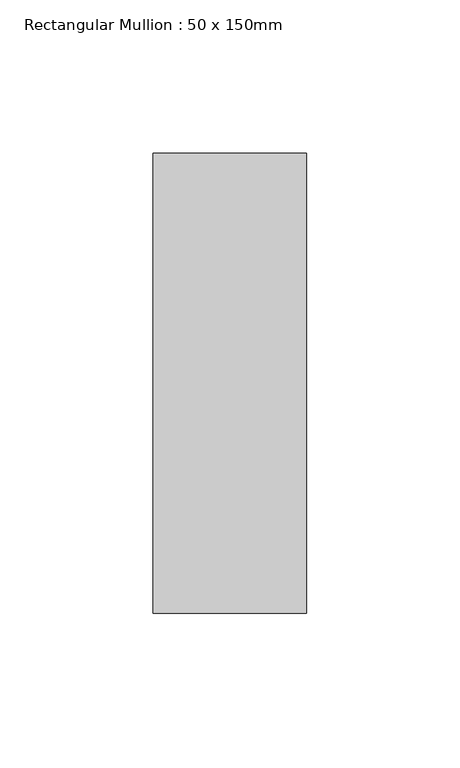
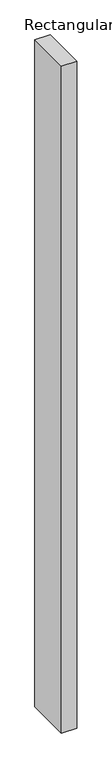
"""IFC4 building model written with IfcOpenShell, lengths in millimetres: member geometry, Rectangular Mullion : 50 x 150mm."""

import ifcopenshell
import ifcopenshell.guid

model = None  # the IFC model being written
_history = None  # IfcOwnerHistory: only IFC2X3 demands one
_inside = {}  # id of a spatial element -> (the spatial element, [elements in it])
_under = {}  # id of a project, library or spatial element -> (it, [spatial elements below it])
_declared = {}  # id of a project -> (the project, [libraries it declares])
_typed = {}  # id of a type object -> (the type object, [elements of that type])
_made_of = {}  # id of a material, layer set ... -> (it, [elements and type objects made of it])


def new_model(schema):
    """Start an empty IFC model of exactly this schema.

    Asked for "IFC4X3", IfcOpenShell would pick the latest addendum, in which some entities
    have other attributes; the version numbers below select the first issue.
    IFC2X3 requires an IfcOwnerHistory on every rooted entity: one is made here for all.
    """
    global model, _history
    if schema == "IFC4X3":
        model = ifcopenshell.file(schema_version=(4, 3, 0, 0))
    else:
        model = ifcopenshell.file(schema=schema)
    _inside.clear()
    _under.clear()
    _declared.clear()
    _typed.clear()
    _made_of.clear()
    _history = None
    if model.schema == "IFC2X3":
        org = make("IfcOrganization", Name="unknown")
        user = make(
            "IfcPersonAndOrganization",
            ThePerson=make("IfcPerson", FamilyName="unknown"),
            TheOrganization=org,
        )
        app = make(
            "IfcApplication",
            ApplicationDeveloper=org,
            Version="unknown",
            ApplicationFullName="unknown",
            ApplicationIdentifier="unknown",
        )
        _history = make(
            "IfcOwnerHistory",
            OwningUser=user,
            OwningApplication=app,
            ChangeAction="ADDED",
            CreationDate=0,
        )
    return model


def make(cls, **values):
    """One entity of the class cls with the attributes given. An attribute that is None is left unset."""
    return model.create_entity(
        cls, **{name: value for name, value in values.items() if value is not None}
    )


def rooted(cls, **values):
    """An entity with a GlobalId (a new one), such as an element, a storey or a relation."""
    return make(cls, GlobalId=ifcopenshell.guid.new(), OwnerHistory=_history, **values)


def si_unit(unit_type, name, prefix=None):
    """IfcSIUnit, for example si_unit("LENGTHUNIT", "METRE", prefix="MILLI")."""
    return make("IfcSIUnit", UnitType=unit_type, Prefix=prefix, Name=name)


def assignment(units):
    """IfcUnitAssignment: the units of a project."""
    return None if units is None else make("IfcUnitAssignment", Units=units)


def point(xyz):
    """IfcCartesianPoint."""
    return None if xyz is None else make("IfcCartesianPoint", Coordinates=xyz)


def direction(xyz):
    """IfcDirection."""
    return None if xyz is None else make("IfcDirection", DirectionRatios=xyz)


def frame(location, z_axis=None, x_axis=None):
    """IfcAxis2Placement3D, a coordinate frame: its origin and axes. An axis left out is left unset."""
    return make(
        "IfcAxis2Placement3D",
        Location=point(location),
        Axis=direction(z_axis),
        RefDirection=direction(x_axis),
    )


def origin():
    """The frame at (0, 0, 0) with its axes left unset."""
    return frame((0.0, 0.0, 0.0))


def place(relative_to, where):
    """IfcLocalPlacement: puts the frame where relative to a parent placement (None: the world)."""
    return make(
        "IfcLocalPlacement", PlacementRelTo=relative_to, RelativePlacement=where
    )


def context(
    kind, dimensions, precision=None, world=None, true_north=None, identifier=None
):
    """IfcGeometricRepresentationContext, for example the 3D "Model" context."""
    return make(
        "IfcGeometricRepresentationContext",
        ContextIdentifier=identifier,
        ContextType=kind,
        CoordinateSpaceDimension=dimensions,
        Precision=precision,
        WorldCoordinateSystem=world,
        TrueNorth=true_north,
    )


def project(units=None, contexts=None):
    """IfcProject with its units and contexts."""
    return rooted(
        "IfcProject",
        Name="project",
        RepresentationContexts=contexts,
        UnitsInContext=assignment(units),
    )


def spatial(cls, under=None, at=None, **own):
    """A site, building, storey or space (cls), placed at a placement, below another one or the project."""
    s = rooted(cls, ObjectPlacement=at, **own)
    if under is not None:
        _under.setdefault(under.id(), (under, []))[1].append(s)
    return s


def polyline(points):
    """IfcPolyline through the points."""
    return make("IfcPolyline", Points=[point(p) for p in points])


def outline(outer, holes=None, kind="AREA"):
    """IfcArbitraryClosedProfileDef: a profile drawn as a closed curve; with holes, ...WithVoids."""
    if holes is None:
        return make("IfcArbitraryClosedProfileDef", ProfileType=kind, OuterCurve=outer)
    return make(
        "IfcArbitraryProfileDefWithVoids",
        ProfileType=kind,
        OuterCurve=outer,
        InnerCurves=holes,
    )


def extrude(swept, where, along, depth):
    """IfcExtrudedAreaSolid: the profile swept, set in the frame where, extruded along a direction by depth."""
    return make(
        "IfcExtrudedAreaSolid",
        SweptArea=swept,
        Position=where,
        ExtrudedDirection=direction(along),
        Depth=depth,
    )


def shape(context_of_items, identifier, shape_type, items):
    """IfcShapeRepresentation: the items that make up one representation, for example the "Body"."""
    return make(
        "IfcShapeRepresentation",
        ContextOfItems=context_of_items,
        RepresentationIdentifier=identifier,
        RepresentationType=shape_type,
        Items=items,
    )


def source(mapping_origin, context_of_items, identifier, shape_type, items):
    """IfcRepresentationMap: a shape defined once, which mapped items show again and again."""
    return make(
        "IfcRepresentationMap",
        MappingOrigin=mapping_origin,
        MappedRepresentation=shape(context_of_items, identifier, shape_type, items),
    )


def transform(
    local_origin,
    x_axis=None,
    y_axis=None,
    z_axis=None,
    scale=None,
    scale2=None,
    scale3=None,
    uniform=True,
):
    """IfcCartesianTransformationOperator3D, or its non-uniform kind. x_axis, y_axis, z_axis: its Axis1, 2, 3."""
    if uniform:
        return make(
            "IfcCartesianTransformationOperator3D",
            Axis1=direction(x_axis),
            Axis2=direction(y_axis),
            LocalOrigin=point(local_origin),
            Scale=scale,
            Axis3=direction(z_axis),
        )
    return make(
        "IfcCartesianTransformationOperator3DnonUniform",
        Axis1=direction(x_axis),
        Axis2=direction(y_axis),
        LocalOrigin=point(local_origin),
        Scale=scale,
        Axis3=direction(z_axis),
        Scale2=scale2,
        Scale3=scale3,
    )


def mapped(mapping_source, mapping_target):
    """IfcMappedItem: shows the shape of a source again, moved by a transform."""
    return make(
        "IfcMappedItem", MappingSource=mapping_source, MappingTarget=mapping_target
    )


def made_of(thing, what):
    """Note that an element or type object is made of a material, layer set ...; save() writes the relation."""
    if what is not None:
        _made_of.setdefault(what.id(), (what, []))[1].append(thing)
    return thing


def element(
    cls,
    number,
    at=None,
    inside=None,
    cuts=None,
    type_object=None,
    material=None,
    context=None,
    identifier="Body",
    shape_type=None,
    held_by="IfcProductDefinitionShape",
    body=None,
    shapes=None,
    **own,
):
    """One element of the class cls, such as IfcWall. Its Tag is "e" and its number.

    at: its placement. inside: the storey or other place that contains it. cuts: it is an
    opening in that element (IfcRelVoidsElement). A single representation is given by context,
    identifier, shape_type and body (its items); several are given by shapes. held_by: the class
    of the entity that holds the representations. save() writes the other relations.
    """
    e = rooted(cls, Tag="e%d" % number, ObjectPlacement=at, **own)
    if body is not None:
        shapes = [shape(context, identifier, shape_type, body)]
    if shapes is not None:
        e.Representation = make(held_by, Representations=shapes)
    if inside is not None:
        _inside.setdefault(inside.id(), (inside, []))[1].append(e)
    if cuts is not None:
        rooted(
            "IfcRelVoidsElement", RelatingBuildingElement=cuts, RelatedOpeningElement=e
        )
    if type_object is not None:
        _typed.setdefault(type_object.id(), (type_object, []))[1].append(e)
    return made_of(e, material)


def aggregate(whole, parts):
    """IfcRelAggregates: a whole, such as a stair, and the parts it consists of."""
    return rooted("IfcRelAggregates", RelatingObject=whole, RelatedObjects=parts)


def save(model, path):
    """Write the relations noted so far, then the file.

    IfcRelAggregates (storeys below a building ...), IfcRelContainedInSpatialStructure (elements
    in a storey), IfcRelDefinesByType, IfcRelAssociatesMaterial and IfcRelDeclares: one each for
    every whole, place, type object, material and project.
    """
    for whole, parts in _under.values():
        aggregate(whole, parts)
    for where, things in _inside.values():
        rooted(
            "IfcRelContainedInSpatialStructure",
            RelatedElements=things,
            RelatingStructure=where,
        )
    for kind, things in _typed.values():
        rooted("IfcRelDefinesByType", RelatedObjects=things, RelatingType=kind)
    for what, things in _made_of.values():
        rooted("IfcRelAssociatesMaterial", RelatedObjects=things, RelatingMaterial=what)
    for by, libraries in _declared.values():
        rooted("IfcRelDeclares", RelatingContext=by, RelatedDefinitions=libraries)
    model.write(path)


def rectangular_mullion_50_x_150mm_8753ce05(model_context):
    return source(origin(), model_context, "Body", "SweptSolid", [
        extrude(outline(polyline([(0.0, 75.0), (0.0, -75.0), (-50.0, -75.0), (-50.0, 75.0), (0.0, 75.0)])), frame((0.0, 0.0, -2300.0), z_axis=(0.0, 0.0, 1.0), x_axis=(1.0, 0.0, 0.0)), (0.0, 0.0, 1.0), 2300.0),
    ])


if __name__ == "__main__":
    model = new_model("IFC4")
    model_context = context("Model", 3, world=origin())
    ifc_project = project(units=[si_unit("LENGTHUNIT", "METRE", prefix="MILLI")], contexts=[model_context])
    site = spatial("IfcSite", under=ifc_project)
    building = spatial("IfcBuilding", under=site)
    placement = place(None, origin())
    rectangular_mullion_50_x_150mm_shape = rectangular_mullion_50_x_150mm_8753ce05(model_context)
    element("IfcMember", 1, ObjectType="Rectangular Mullion : 50 x 150mm", at=placement, inside=building, context=model_context, shape_type="MappedRepresentation", body=[
        mapped(rectangular_mullion_50_x_150mm_shape, transform((0.0, 0.0, 0.0), x_axis=(1.0, 0.0, 0.0), y_axis=(0.0, 1.0, 0.0), z_axis=(0.0, 0.0, 1.0))),
    ])
    save(model, "model.ifc")

# Revit data of these elements
# Type "Rectangular Mullion : 50 x 150mm"
#   built-in parameter 1007304 = 0.492126 (stored number, unit not read)
#   built-in parameter 1007301 = 0.082021 (stored number, unit not read)
#   built-in parameter 1007300 = 0.082021 (stored number, unit not read)
# Element 1 (IfcMember, "Rectangular Mullion : 50 x 150mm")
#   Materials on its faces: "Metal - Aluminium"
# Materials
#   "Metal - Aluminium": class "Metal", colour RGB 247 247 247, transparency 0
